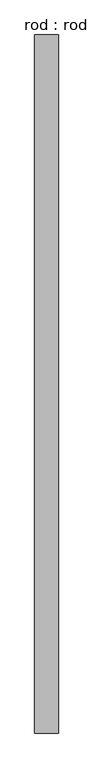
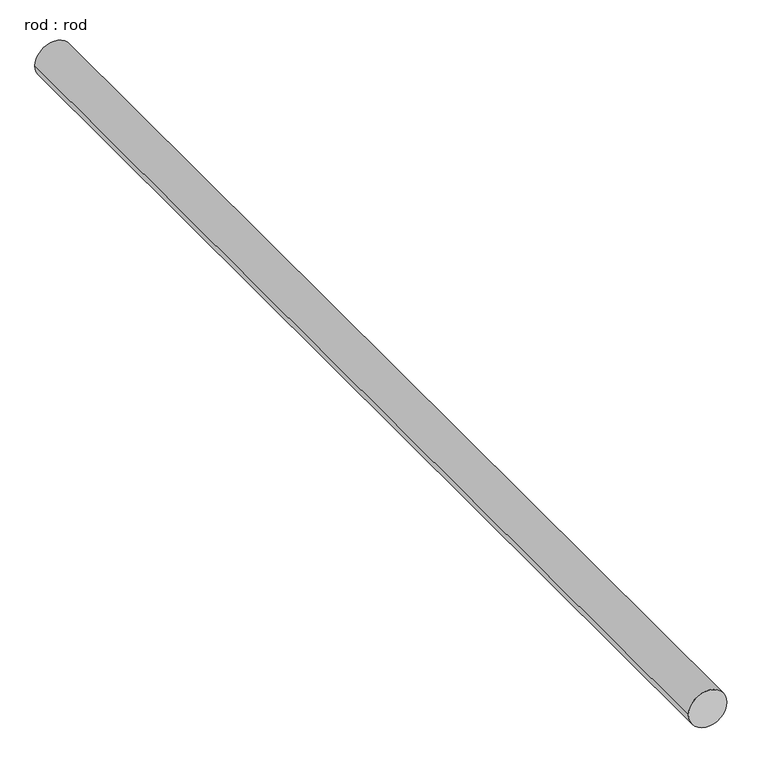
"""IFC4 building model written with IfcOpenShell, lengths in millimetres: proxy geometry, rod : rod."""

from ifc_helpers import new_model, si_unit, point, frame, frame_2d, origin, place, context, project, spatial, circle_curve, trimmed, segment, composite_curve, outline, extrude, source, transform, mapped, element, save


def rod_rod_c80f3376(model_context):
    return source(origin(), model_context, "Body", "SweptSolid", [
        extrude(outline(composite_curve([segment(trimmed(circle_curve(frame_2d((0.0108462, 0.0)), 200.0), [point((0.0108462, 200.0))], [point((0.0108462, -200.0))], False, "CARTESIAN"), True, "CONTINUOUS"), segment(trimmed(circle_curve(frame_2d((0.0108462, 0.0)), 200.0), [point((0.0108462, -200.0))], [point((0.0108462, 200.0))], False, "CARTESIAN"), True, "CONTINUOUS")], self_intersect=False)), frame((0.0, -1823.9380513, 0.0), z_axis=(0.0, 1.0, 0.0), x_axis=(0.0, 0.0, 1.0)), (0.0, 0.0, 1.0), 11833.3333333),
    ])


if __name__ == "__main__":
    model = new_model("IFC4")
    model_context = context("Model", 3, world=origin())
    ifc_project = project(units=[si_unit("LENGTHUNIT", "METRE", prefix="MILLI")], contexts=[model_context])
    site = spatial("IfcSite", under=ifc_project)
    building = spatial("IfcBuilding", under=site)
    placement = place(None, origin())
    rod_rod_shape = rod_rod_c80f3376(model_context)
    element("IfcBuildingElementProxy", 1, Name="rod : rod", ObjectType="rod : rod", at=placement, inside=building, context=model_context, shape_type="MappedRepresentation", body=[
        mapped(rod_rod_shape, transform((0.0, 0.0, 0.0), x_axis=(1.0, 0.0, 0.0), y_axis=(0.0, 1.0, 0.0), z_axis=(0.0, 0.0, 1.0))),
    ])
    save(model, "model.ifc")

# Revit data of these elements
# Type "rod : rod"
#   Default Elevation = 0
